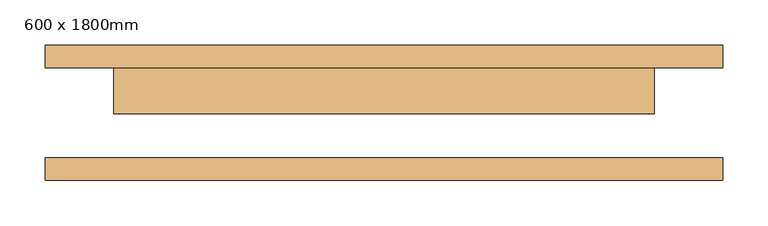
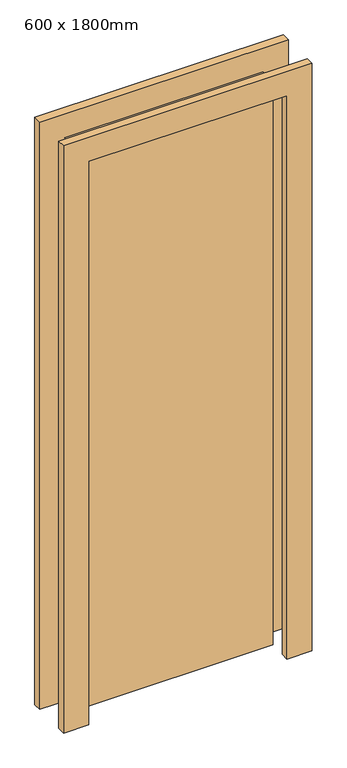
"""IFC4 building model written with IfcOpenShell, lengths in millimetres: door geometry, 单扇 - 与墙齐 : 600 x 1800mm."""

import ifcopenshell
import ifcopenshell.guid

model = None  # the IFC model being written
_history = None  # IfcOwnerHistory: only IFC2X3 demands one
_inside = {}  # id of a spatial element -> (the spatial element, [elements in it])
_under = {}  # id of a project, library or spatial element -> (it, [spatial elements below it])
_declared = {}  # id of a project -> (the project, [libraries it declares])
_typed = {}  # id of a type object -> (the type object, [elements of that type])
_made_of = {}  # id of a material, layer set ... -> (it, [elements and type objects made of it])


def new_model(schema):
    """Start an empty IFC model of exactly this schema.

    Asked for "IFC4X3", IfcOpenShell would pick the latest addendum, in which some entities
    have other attributes; the version numbers below select the first issue.
    IFC2X3 requires an IfcOwnerHistory on every rooted entity: one is made here for all.
    """
    global model, _history
    if schema == "IFC4X3":
        model = ifcopenshell.file(schema_version=(4, 3, 0, 0))
    else:
        model = ifcopenshell.file(schema=schema)
    _inside.clear()
    _under.clear()
    _declared.clear()
    _typed.clear()
    _made_of.clear()
    _history = None
    if model.schema == "IFC2X3":
        org = make("IfcOrganization", Name="unknown")
        user = make(
            "IfcPersonAndOrganization",
            ThePerson=make("IfcPerson", FamilyName="unknown"),
            TheOrganization=org,
        )
        app = make(
            "IfcApplication",
            ApplicationDeveloper=org,
            Version="unknown",
            ApplicationFullName="unknown",
            ApplicationIdentifier="unknown",
        )
        _history = make(
            "IfcOwnerHistory",
            OwningUser=user,
            OwningApplication=app,
            ChangeAction="ADDED",
            CreationDate=0,
        )
    return model


def make(cls, **values):
    """One entity of the class cls with the attributes given. An attribute that is None is left unset."""
    return model.create_entity(
        cls, **{name: value for name, value in values.items() if value is not None}
    )


def rooted(cls, **values):
    """An entity with a GlobalId (a new one), such as an element, a storey or a relation."""
    return make(cls, GlobalId=ifcopenshell.guid.new(), OwnerHistory=_history, **values)


def si_unit(unit_type, name, prefix=None):
    """IfcSIUnit, for example si_unit("LENGTHUNIT", "METRE", prefix="MILLI")."""
    return make("IfcSIUnit", UnitType=unit_type, Prefix=prefix, Name=name)


def assignment(units):
    """IfcUnitAssignment: the units of a project."""
    return None if units is None else make("IfcUnitAssignment", Units=units)


def point(xyz):
    """IfcCartesianPoint."""
    return None if xyz is None else make("IfcCartesianPoint", Coordinates=xyz)


def direction(xyz):
    """IfcDirection."""
    return None if xyz is None else make("IfcDirection", DirectionRatios=xyz)


def frame(location, z_axis=None, x_axis=None):
    """IfcAxis2Placement3D, a coordinate frame: its origin and axes. An axis left out is left unset."""
    return make(
        "IfcAxis2Placement3D",
        Location=point(location),
        Axis=direction(z_axis),
        RefDirection=direction(x_axis),
    )


def origin():
    """The frame at (0, 0, 0) with its axes left unset."""
    return frame((0.0, 0.0, 0.0))


def origin_with_axes():
    """The frame at (0, 0, 0) with the z axis (0, 0, 1) and the x axis (1, 0, 0) written out."""
    return frame((0.0, 0.0, 0.0), z_axis=(0.0, 0.0, 1.0), x_axis=(1.0, 0.0, 0.0))


def place(relative_to, where):
    """IfcLocalPlacement: puts the frame where relative to a parent placement (None: the world)."""
    return make(
        "IfcLocalPlacement", PlacementRelTo=relative_to, RelativePlacement=where
    )


def context(
    kind, dimensions, precision=None, world=None, true_north=None, identifier=None
):
    """IfcGeometricRepresentationContext, for example the 3D "Model" context."""
    return make(
        "IfcGeometricRepresentationContext",
        ContextIdentifier=identifier,
        ContextType=kind,
        CoordinateSpaceDimension=dimensions,
        Precision=precision,
        WorldCoordinateSystem=world,
        TrueNorth=true_north,
    )


def project(units=None, contexts=None):
    """IfcProject with its units and contexts."""
    return rooted(
        "IfcProject",
        Name="project",
        RepresentationContexts=contexts,
        UnitsInContext=assignment(units),
    )


def spatial(cls, under=None, at=None, **own):
    """A site, building, storey or space (cls), placed at a placement, below another one or the project."""
    s = rooted(cls, ObjectPlacement=at, **own)
    if under is not None:
        _under.setdefault(under.id(), (under, []))[1].append(s)
    return s


def polyline(points):
    """IfcPolyline through the points."""
    return make("IfcPolyline", Points=[point(p) for p in points])


def outline(outer, holes=None, kind="AREA"):
    """IfcArbitraryClosedProfileDef: a profile drawn as a closed curve; with holes, ...WithVoids."""
    if holes is None:
        return make("IfcArbitraryClosedProfileDef", ProfileType=kind, OuterCurve=outer)
    return make(
        "IfcArbitraryProfileDefWithVoids",
        ProfileType=kind,
        OuterCurve=outer,
        InnerCurves=holes,
    )


def extrude(swept, where, along, depth):
    """IfcExtrudedAreaSolid: the profile swept, set in the frame where, extruded along a direction by depth."""
    return make(
        "IfcExtrudedAreaSolid",
        SweptArea=swept,
        Position=where,
        ExtrudedDirection=direction(along),
        Depth=depth,
    )


def shape(context_of_items, identifier, shape_type, items):
    """IfcShapeRepresentation: the items that make up one representation, for example the "Body"."""
    return make(
        "IfcShapeRepresentation",
        ContextOfItems=context_of_items,
        RepresentationIdentifier=identifier,
        RepresentationType=shape_type,
        Items=items,
    )


def source(mapping_origin, context_of_items, identifier, shape_type, items):
    """IfcRepresentationMap: a shape defined once, which mapped items show again and again."""
    return make(
        "IfcRepresentationMap",
        MappingOrigin=mapping_origin,
        MappedRepresentation=shape(context_of_items, identifier, shape_type, items),
    )


def transform(
    local_origin,
    x_axis=None,
    y_axis=None,
    z_axis=None,
    scale=None,
    scale2=None,
    scale3=None,
    uniform=True,
):
    """IfcCartesianTransformationOperator3D, or its non-uniform kind. x_axis, y_axis, z_axis: its Axis1, 2, 3."""
    if uniform:
        return make(
            "IfcCartesianTransformationOperator3D",
            Axis1=direction(x_axis),
            Axis2=direction(y_axis),
            LocalOrigin=point(local_origin),
            Scale=scale,
            Axis3=direction(z_axis),
        )
    return make(
        "IfcCartesianTransformationOperator3DnonUniform",
        Axis1=direction(x_axis),
        Axis2=direction(y_axis),
        LocalOrigin=point(local_origin),
        Scale=scale,
        Axis3=direction(z_axis),
        Scale2=scale2,
        Scale3=scale3,
    )


def mapped(mapping_source, mapping_target):
    """IfcMappedItem: shows the shape of a source again, moved by a transform."""
    return make(
        "IfcMappedItem", MappingSource=mapping_source, MappingTarget=mapping_target
    )


def made_of(thing, what):
    """Note that an element or type object is made of a material, layer set ...; save() writes the relation."""
    if what is not None:
        _made_of.setdefault(what.id(), (what, []))[1].append(thing)
    return thing


def element(
    cls,
    number,
    at=None,
    inside=None,
    cuts=None,
    type_object=None,
    material=None,
    context=None,
    identifier="Body",
    shape_type=None,
    held_by="IfcProductDefinitionShape",
    body=None,
    shapes=None,
    **own,
):
    """One element of the class cls, such as IfcWall. Its Tag is "e" and its number.

    at: its placement. inside: the storey or other place that contains it. cuts: it is an
    opening in that element (IfcRelVoidsElement). A single representation is given by context,
    identifier, shape_type and body (its items); several are given by shapes. held_by: the class
    of the entity that holds the representations. save() writes the other relations.
    """
    e = rooted(cls, Tag="e%d" % number, ObjectPlacement=at, **own)
    if body is not None:
        shapes = [shape(context, identifier, shape_type, body)]
    if shapes is not None:
        e.Representation = make(held_by, Representations=shapes)
    if inside is not None:
        _inside.setdefault(inside.id(), (inside, []))[1].append(e)
    if cuts is not None:
        rooted(
            "IfcRelVoidsElement", RelatingBuildingElement=cuts, RelatedOpeningElement=e
        )
    if type_object is not None:
        _typed.setdefault(type_object.id(), (type_object, []))[1].append(e)
    return made_of(e, material)


def aggregate(whole, parts):
    """IfcRelAggregates: a whole, such as a stair, and the parts it consists of."""
    return rooted("IfcRelAggregates", RelatingObject=whole, RelatedObjects=parts)


def save(model, path):
    """Write the relations noted so far, then the file.

    IfcRelAggregates (storeys below a building ...), IfcRelContainedInSpatialStructure (elements
    in a storey), IfcRelDefinesByType, IfcRelAssociatesMaterial and IfcRelDeclares: one each for
    every whole, place, type object, material and project.
    """
    for whole, parts in _under.values():
        aggregate(whole, parts)
    for where, things in _inside.values():
        rooted(
            "IfcRelContainedInSpatialStructure",
            RelatedElements=things,
            RelatingStructure=where,
        )
    for kind, things in _typed.values():
        rooted("IfcRelDefinesByType", RelatedObjects=things, RelatingType=kind)
    for what, things in _made_of.values():
        rooted("IfcRelAssociatesMaterial", RelatedObjects=things, RelatingMaterial=what)
    for by, libraries in _declared.values():
        rooted("IfcRelDeclares", RelatingContext=by, RelatedDefinitions=libraries)
    model.write(path)


def door_600_x_1800mm_79ebe2d6(model_context):
    return source(origin(), model_context, "Body", "SweptSolid", [
        extrude(outline(polyline([(1876.0, -376.0), (0.0, -376.0), (0.0, -300.0), (1800.0, -300.0), (1800.0, 300.0), (0.0, 300.0), (0.0, 376.0), (1876.0, 376.0), (1876.0, -376.0)])), frame((0.0, 50.0, 0.0), z_axis=(0.0, 1.0, 0.0), x_axis=(0.0, 0.0, 1.0)), (0.0, 0.0, 1.0), 25.0),
        extrude(outline(polyline([(1876.0, 376.0), (1876.0, -376.0), (0.0, -376.0), (0.0, -300.0), (1800.0, -300.0), (1800.0, 300.0), (0.0, 300.0), (0.0, 376.0), (1876.0, 376.0)])), frame((0.0, -75.0, 0.0), z_axis=(0.0, 1.0, 0.0), x_axis=(0.0, 0.0, 1.0)), (0.0, 0.0, 1.0), 25.0),
        extrude(outline(polyline([(300.0, -1.0), (-300.0, -1.0), (-300.0, 50.0), (300.0, 50.0), (300.0, -1.0)])), origin_with_axes(), (0.0, 0.0, 1.0), 1800.0),
    ])


if __name__ == "__main__":
    model = new_model("IFC4")
    model_context = context("Model", 3, world=origin())
    ifc_project = project(units=[si_unit("LENGTHUNIT", "METRE", prefix="MILLI")], contexts=[model_context])
    site = spatial("IfcSite", under=ifc_project)
    building = spatial("IfcBuilding", under=site)
    placement = place(None, origin())
    door_600_x_1800mm_shape = door_600_x_1800mm_79ebe2d6(model_context)
    element("IfcDoor", 1, ObjectType="单扇 - 与墙齐 : 600 x 1800mm", at=placement, inside=building, context=model_context, shape_type="MappedRepresentation", body=[
        mapped(door_600_x_1800mm_shape, transform((0.0, 0.0, 0.0), x_axis=(1.0, 0.0, 0.0), y_axis=(0.0, 1.0, 0.0), z_axis=(0.0, 0.0, 1.0))),
    ])
    save(model, "model.ifc")

# Revit data of these elements
# Type "单扇 - 与墙齐 : 600 x 1800mm"
#   Type Mark = "M0618"
#   Construction Type Id = "MDOOR"
#   Analytic Construction = "金属"
#   贴面宽度 = 76 mm
#   贴面投影内部 = 25 mm
#   贴面投影外部 = 25 mm
#   Thickness = 51 mm
#   Height = 1800 mm
#   Width = 600 mm
#   Heat Transfer Coefficient (U) = 3.7021 W/(m²·K)
#   框架材质 = 门 - 框架
#   门材质 = 门 - 嵌板
#   Visual Light Transmittance = 0
#   Solar Heat Gain Coefficient = 0
#   Wall Closure = (empty or 0)
#   Function = (empty or 0)
# Element 1 (IfcDoor, "单扇 - 与墙齐 : 600 x 1800mm")
#   Materials on its faces: "门 - 框架", "门 - 嵌板"
# Materials
#   "门 - 框架": class "其他", colour RGB 118 70 51, transparency 0, Cost = 0
#   "门 - 嵌板": class "木质", colour RGB 210 159 95, transparency 0, Cost = 0
